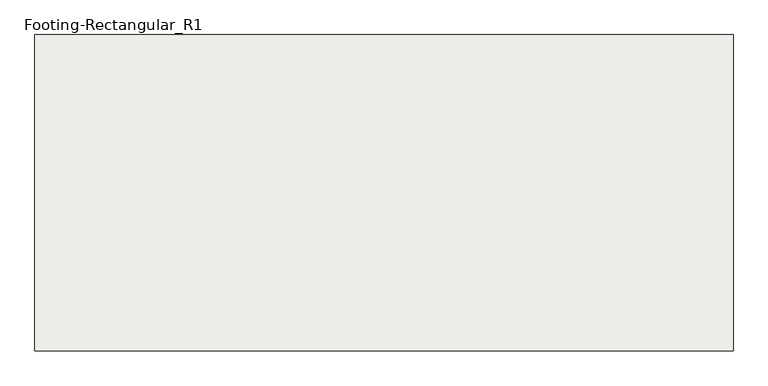
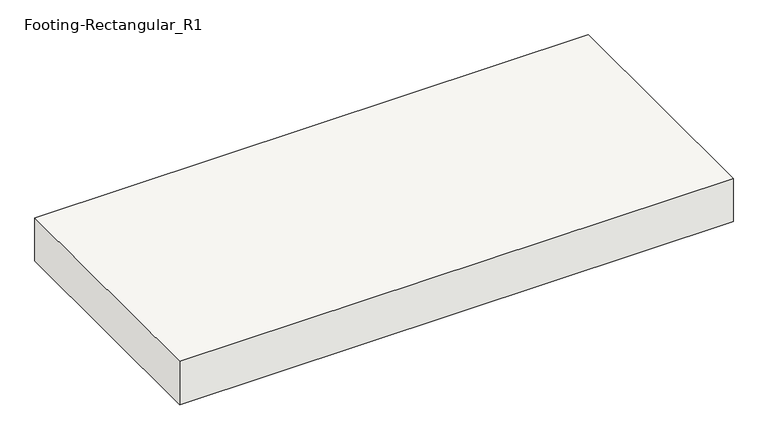
"""IFC4 building model written with IfcOpenShell, lengths in millimetres: slab geometry, Footing-Rectangular_R1 : H_SF_AR_S18_W6050xL2740xT500_Bitumen_F8."""

from ifc_helpers import new_model, si_unit, frame, origin, place, context, project, spatial, polyline, outline, extrude, source, transform, mapped, element, save


def footing_rectangular_r1_8e80394c(model_context):
    return source(origin(), model_context, "Body", "SweptSolid", [
        extrude(outline(polyline([(3025.0, 1370.0), (3025.0, -1370.0), (-3025.0, -1370.0), (-3025.0, 1370.0), (3025.0, 1370.0)])), frame((0.0, 0.0, -500.0), z_axis=(0.0, 0.0, 1.0), x_axis=(1.0, 0.0, 0.0)), (0.0, 0.0, 1.0), 500.0),
    ])


if __name__ == "__main__":
    model = new_model("IFC4")
    model_context = context("Model", 3, world=origin())
    ifc_project = project(units=[si_unit("LENGTHUNIT", "METRE", prefix="MILLI")], contexts=[model_context])
    site = spatial("IfcSite", under=ifc_project)
    building = spatial("IfcBuilding", under=site)
    placement = place(None, origin())
    footing_rectangular_r1_shape = footing_rectangular_r1_8e80394c(model_context)
    element("IfcSlab", 1, ObjectType="Footing-Rectangular_R1 : H_SF_AR_S18_W6050xL2740xT500_Bitumen_F8", at=placement, inside=building, context=model_context, shape_type="MappedRepresentation", body=[
        mapped(footing_rectangular_r1_shape, transform((0.0, 0.0, 0.0), x_axis=(1.0, 0.0, 0.0), y_axis=(0.0, 1.0, 0.0), z_axis=(0.0, 0.0, 1.0))),
    ])
    save(model, "model.ifc")

# Revit data of these elements
# Type "Footing-Rectangular_R1 : H_SF_AR_S18_W6050xL2740xT500_Bitumen_F8"
#   Type Mark = "F8"
#   Top bar = "D25@300"
#   Description = "UG Shallow Foundation"
#   Bottom bar = "D20@300"
#   Width = 6050 mm
#   Length = 2740 mm
#   Foundation Thickness = 500 mm
#   Structural Material [instance default] = none
#   Assembly Code = ""
